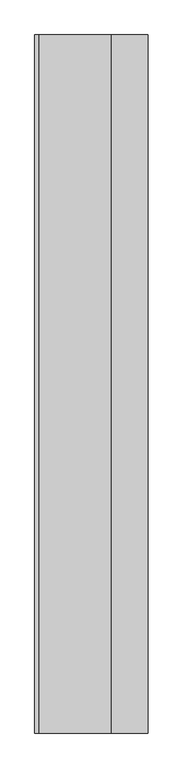
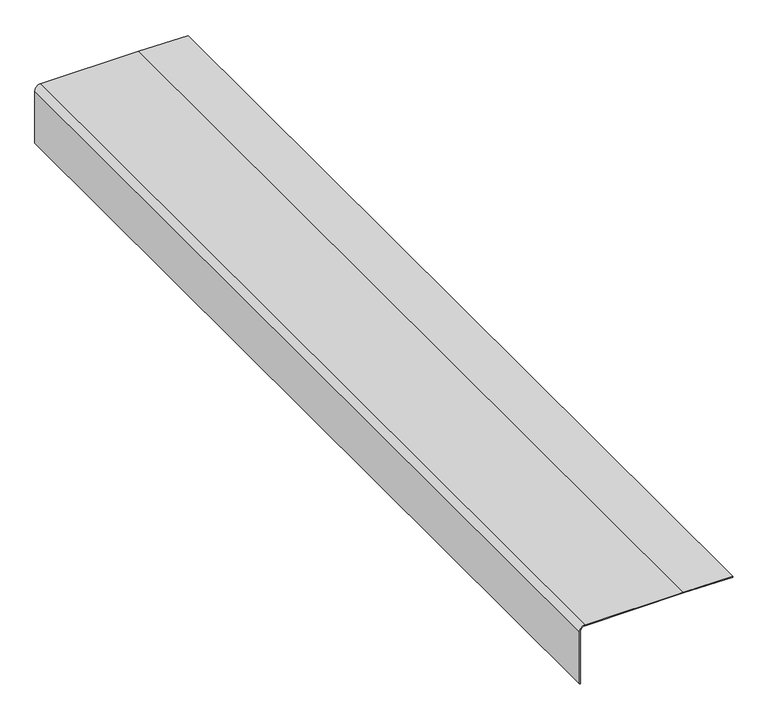
"""IFC4 building model written with IfcOpenShell, lengths in millimetres: proxy geometry, Membrane059 4742 : Membrane059 4742."""

from ifc_helpers import new_model, si_unit, point, frame, frame_2d, origin, place, context, project, spatial, polyline, circle_curve, trimmed, segment, composite_curve, outline, extrude, source, transform, mapped, element, save


def generic_models_4834b2ef(model_context):
    return source(origin(), model_context, "Body", "SweptSolid", [
        extrude(outline(composite_curve([segment(trimmed(circle_curve(frame_2d((40233.3001163, -5012.5056829)), 10.0), [point((40233.3001163, -5022.5056829))], [point((40243.3001163, -5012.5056829))], True, "CARTESIAN"), True, "CONTINUOUS"), segment(polyline([(40243.3001163, -5012.5056829), (40243.3001163, -4804.1710546), (40241.7972226, -4699.8063764), (40243.79743, -4699.8063764), (40245.3001163, -4804.1566552), (40245.3001163, -5012.5056829)]), True, "CONTINUOUS"), segment(trimmed(circle_curve(frame_2d((40233.3001163, -5012.5056829)), 12.0), [point((40245.3001163, -5012.5056829))], [point((40233.3001163, -5024.5056829))], False, "CARTESIAN"), True, "CONTINUOUS"), segment(polyline([(40233.3001163, -5024.5056829), (40116.5801181, -5024.5056829), (40116.5801181, -5022.5056829), (40233.3001163, -5022.5056829)]), True, "CONTINUOUS")], self_intersect=False)), frame((0.0, -1052.8906574, 0.0), z_axis=(0.0, 1.0, 0.0), x_axis=(0.0, 0.0, 1.0)), (0.0, 0.0, 1.0), 2000.0),
    ])


if __name__ == "__main__":
    model = new_model("IFC4")
    model_context = context("Model", 3, world=origin())
    ifc_project = project(units=[si_unit("LENGTHUNIT", "METRE", prefix="MILLI")], contexts=[model_context])
    site = spatial("IfcSite", under=ifc_project)
    building = spatial("IfcBuilding", under=site)
    placement = place(None, origin())
    generic_models_shape = generic_models_4834b2ef(model_context)
    element("IfcBuildingElementProxy", 1, Name="Membrane059 4742 : Membrane059 4742", ObjectType="Membrane059 4742 : Membrane059 4742", at=placement, inside=building, context=model_context, shape_type="MappedRepresentation", body=[
        mapped(generic_models_shape, transform((0.0, 0.0, 0.0), x_axis=(1.0, 0.0, 0.0), y_axis=(0.0, 1.0, 0.0), z_axis=(0.0, 0.0, 1.0))),
    ])
    save(model, "model.ifc")

# Revit data of these elements
# Type "Membrane059 4742 : Membrane059 4742"
#   NameOverride = "Membrane059"
# Element 1 (IfcBuildingElementProxy, "Membrane059 4742 : Membrane059 4742")
#   Materials on its faces: "THREE PLY BUILT UP ROOF MEMBRANE"
# Materials
#   "THREE PLY BUILT UP ROOF MEMBRANE": class "Unassigned", colour RGB 63 63 63, transparency 0
